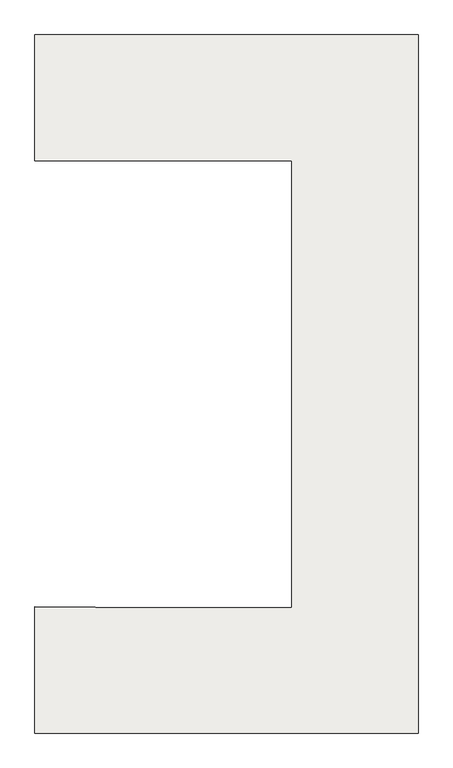
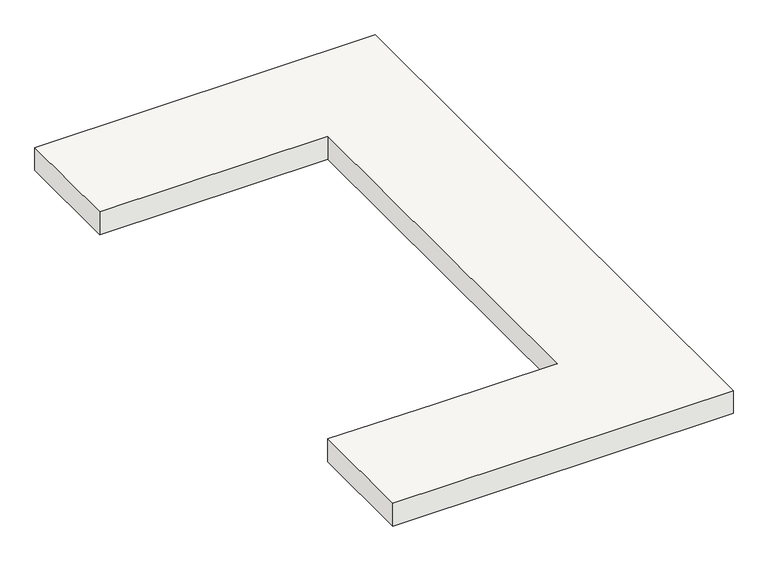
"""IFC4 building model written with IfcOpenShell, lengths in millimetres: slab geometry, Holzdecke."""

from ifc_helpers import new_model, si_unit, origin, origin_with_axes, place, context, project, spatial, polyline, outline, extrude, source, transform, mapped, element, save


def slab_9ff9450e(model_context):
    return source(origin(), model_context, "Body", "SweptSolid", [
        extrude(outline(polyline([(0.0, 5675.0), (0.0, 6925.0), (3800.0, 6925.0), (3800.0, 0.0), (0.0, 0.0), (0.0, 1255.0), (1198.7620124, 1240.7517347), (2550.0, 1240.7517347), (2550.0, 5675.0), (0.0, 5675.0)])), origin_with_axes(), (0.0, 0.0, 1.0), 270.0),
    ])


if __name__ == "__main__":
    model = new_model("IFC4")
    model_context = context("Model", 3, world=origin())
    ifc_project = project(units=[si_unit("LENGTHUNIT", "METRE", prefix="MILLI")], contexts=[model_context])
    site = spatial("IfcSite", under=ifc_project)
    building = spatial("IfcBuilding", under=site)
    placement = place(None, origin())
    slab_shape = slab_9ff9450e(model_context)
    element("IfcSlab", 1, ObjectType="Holzdecke", at=placement, inside=building, context=model_context, shape_type="MappedRepresentation", body=[
        mapped(slab_shape, transform((0.0, 0.0, 0.0), x_axis=(1.0, 0.0, 0.0), y_axis=(0.0, 1.0, 0.0), z_axis=(0.0, 0.0, 1.0))),
    ])
    save(model, "model.ifc")

# Revit data of these elements
# Element 1 (IfcSlab, "Holzdecke")
#   Materials on its faces: "holzschalung"
# Materials
#   "holzschalung": class "Unassigned", colour RGB 128 128 128, transparency 0
